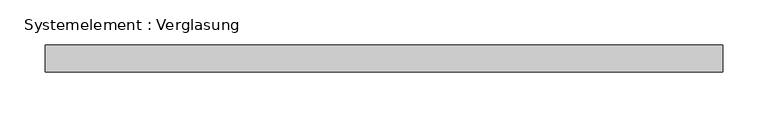
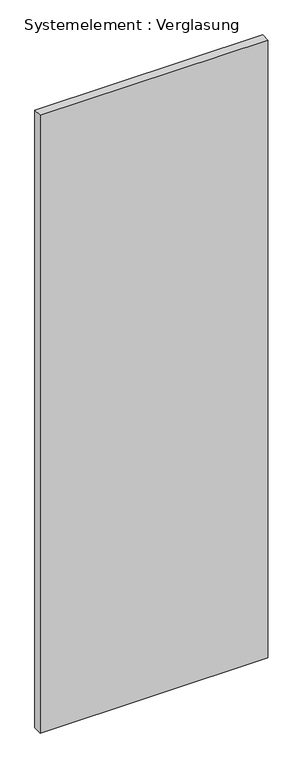
"""IFC4 building model written with IfcOpenShell, lengths in millimetres: plate geometry, Systemelement : Verglasung."""

from ifc_helpers import new_model, si_unit, origin, origin_with_axes, place, context, project, spatial, polyline, outline, extrude, source, transform, mapped, element, save


def systemelement_verglasung_fb34f152(model_context):
    return source(origin(), model_context, "Body", "SweptSolid", [
        extrude(outline(polyline([(376.4731315, -15.0), (-376.4731315, -15.0), (-376.4731315, 15.0), (376.4731315, 15.0), (376.4731315, -15.0)])), origin_with_axes(), (0.0, 0.0, 1.0), 2160.0),
    ])


if __name__ == "__main__":
    model = new_model("IFC4")
    model_context = context("Model", 3, world=origin())
    ifc_project = project(units=[si_unit("LENGTHUNIT", "METRE", prefix="MILLI")], contexts=[model_context])
    site = spatial("IfcSite", under=ifc_project)
    building = spatial("IfcBuilding", under=site)
    placement = place(None, origin())
    systemelement_verglasung_shape = systemelement_verglasung_fb34f152(model_context)
    element("IfcPlate", 1, ObjectType="Systemelement : Verglasung", at=placement, inside=building, context=model_context, shape_type="MappedRepresentation", body=[
        mapped(systemelement_verglasung_shape, transform((0.0, 0.0, 0.0), x_axis=(1.0, 0.0, 0.0), y_axis=(0.0, 1.0, 0.0), z_axis=(0.0, 0.0, 1.0))),
    ])
    save(model, "model.ifc")

# Revit data of these elements
# Type "Systemelement : Verglasung"
#   Construction Type Id = "GSP4R"
#   Analytic Construction = "1/8 Zoll Pilkington-Verglasung einfach"
#   Visual Light Transmittance = 0.9
#   Solar Heat Gain Coefficient = 0.86
#   Heat Transfer Coefficient (U) = 6.7069 W/(m²·K)
# Element 1 (IfcPlate, "Systemelement : Verglasung")
#   Materials on its faces: "Glas"
# Materials
#   "Glas": class "Glas", colour RGB 0 0 255, transparency 0.75, Comments = "Render-Darstellung nicht aktualisiert ", Cost = 0
